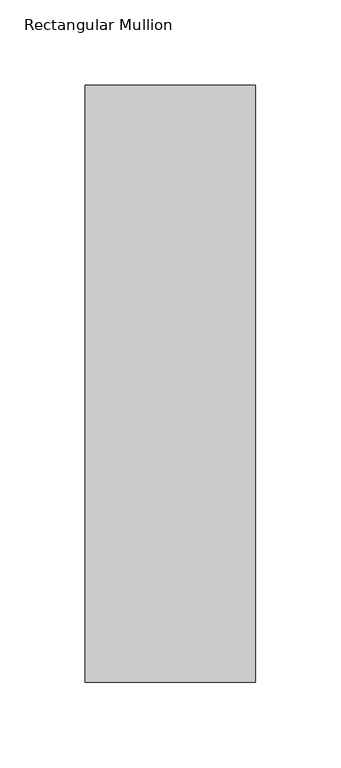
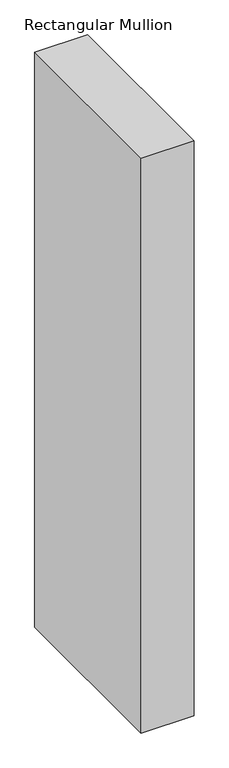
"""IFC4 building model written with IfcOpenShell, lengths in millimetres: member geometry, Rectangular Mullion : WWm-100x350-100mmOffset."""

import ifcopenshell
import ifcopenshell.guid

model = None  # the IFC model being written
_history = None  # IfcOwnerHistory: only IFC2X3 demands one
_inside = {}  # id of a spatial element -> (the spatial element, [elements in it])
_under = {}  # id of a project, library or spatial element -> (it, [spatial elements below it])
_declared = {}  # id of a project -> (the project, [libraries it declares])
_typed = {}  # id of a type object -> (the type object, [elements of that type])
_made_of = {}  # id of a material, layer set ... -> (it, [elements and type objects made of it])


def new_model(schema):
    """Start an empty IFC model of exactly this schema.

    Asked for "IFC4X3", IfcOpenShell would pick the latest addendum, in which some entities
    have other attributes; the version numbers below select the first issue.
    IFC2X3 requires an IfcOwnerHistory on every rooted entity: one is made here for all.
    """
    global model, _history
    if schema == "IFC4X3":
        model = ifcopenshell.file(schema_version=(4, 3, 0, 0))
    else:
        model = ifcopenshell.file(schema=schema)
    _inside.clear()
    _under.clear()
    _declared.clear()
    _typed.clear()
    _made_of.clear()
    _history = None
    if model.schema == "IFC2X3":
        org = make("IfcOrganization", Name="unknown")
        user = make(
            "IfcPersonAndOrganization",
            ThePerson=make("IfcPerson", FamilyName="unknown"),
            TheOrganization=org,
        )
        app = make(
            "IfcApplication",
            ApplicationDeveloper=org,
            Version="unknown",
            ApplicationFullName="unknown",
            ApplicationIdentifier="unknown",
        )
        _history = make(
            "IfcOwnerHistory",
            OwningUser=user,
            OwningApplication=app,
            ChangeAction="ADDED",
            CreationDate=0,
        )
    return model


def make(cls, **values):
    """One entity of the class cls with the attributes given. An attribute that is None is left unset."""
    return model.create_entity(
        cls, **{name: value for name, value in values.items() if value is not None}
    )


def rooted(cls, **values):
    """An entity with a GlobalId (a new one), such as an element, a storey or a relation."""
    return make(cls, GlobalId=ifcopenshell.guid.new(), OwnerHistory=_history, **values)


def si_unit(unit_type, name, prefix=None):
    """IfcSIUnit, for example si_unit("LENGTHUNIT", "METRE", prefix="MILLI")."""
    return make("IfcSIUnit", UnitType=unit_type, Prefix=prefix, Name=name)


def assignment(units):
    """IfcUnitAssignment: the units of a project."""
    return None if units is None else make("IfcUnitAssignment", Units=units)


def point(xyz):
    """IfcCartesianPoint."""
    return None if xyz is None else make("IfcCartesianPoint", Coordinates=xyz)


def direction(xyz):
    """IfcDirection."""
    return None if xyz is None else make("IfcDirection", DirectionRatios=xyz)


def frame(location, z_axis=None, x_axis=None):
    """IfcAxis2Placement3D, a coordinate frame: its origin and axes. An axis left out is left unset."""
    return make(
        "IfcAxis2Placement3D",
        Location=point(location),
        Axis=direction(z_axis),
        RefDirection=direction(x_axis),
    )


def origin():
    """The frame at (0, 0, 0) with its axes left unset."""
    return frame((0.0, 0.0, 0.0))


def place(relative_to, where):
    """IfcLocalPlacement: puts the frame where relative to a parent placement (None: the world)."""
    return make(
        "IfcLocalPlacement", PlacementRelTo=relative_to, RelativePlacement=where
    )


def context(
    kind, dimensions, precision=None, world=None, true_north=None, identifier=None
):
    """IfcGeometricRepresentationContext, for example the 3D "Model" context."""
    return make(
        "IfcGeometricRepresentationContext",
        ContextIdentifier=identifier,
        ContextType=kind,
        CoordinateSpaceDimension=dimensions,
        Precision=precision,
        WorldCoordinateSystem=world,
        TrueNorth=true_north,
    )


def project(units=None, contexts=None):
    """IfcProject with its units and contexts."""
    return rooted(
        "IfcProject",
        Name="project",
        RepresentationContexts=contexts,
        UnitsInContext=assignment(units),
    )


def spatial(cls, under=None, at=None, **own):
    """A site, building, storey or space (cls), placed at a placement, below another one or the project."""
    s = rooted(cls, ObjectPlacement=at, **own)
    if under is not None:
        _under.setdefault(under.id(), (under, []))[1].append(s)
    return s


def polyline(points):
    """IfcPolyline through the points."""
    return make("IfcPolyline", Points=[point(p) for p in points])


def outline(outer, holes=None, kind="AREA"):
    """IfcArbitraryClosedProfileDef: a profile drawn as a closed curve; with holes, ...WithVoids."""
    if holes is None:
        return make("IfcArbitraryClosedProfileDef", ProfileType=kind, OuterCurve=outer)
    return make(
        "IfcArbitraryProfileDefWithVoids",
        ProfileType=kind,
        OuterCurve=outer,
        InnerCurves=holes,
    )


def extrude(swept, where, along, depth):
    """IfcExtrudedAreaSolid: the profile swept, set in the frame where, extruded along a direction by depth."""
    return make(
        "IfcExtrudedAreaSolid",
        SweptArea=swept,
        Position=where,
        ExtrudedDirection=direction(along),
        Depth=depth,
    )


def shape(context_of_items, identifier, shape_type, items):
    """IfcShapeRepresentation: the items that make up one representation, for example the "Body"."""
    return make(
        "IfcShapeRepresentation",
        ContextOfItems=context_of_items,
        RepresentationIdentifier=identifier,
        RepresentationType=shape_type,
        Items=items,
    )


def source(mapping_origin, context_of_items, identifier, shape_type, items):
    """IfcRepresentationMap: a shape defined once, which mapped items show again and again."""
    return make(
        "IfcRepresentationMap",
        MappingOrigin=mapping_origin,
        MappedRepresentation=shape(context_of_items, identifier, shape_type, items),
    )


def transform(
    local_origin,
    x_axis=None,
    y_axis=None,
    z_axis=None,
    scale=None,
    scale2=None,
    scale3=None,
    uniform=True,
):
    """IfcCartesianTransformationOperator3D, or its non-uniform kind. x_axis, y_axis, z_axis: its Axis1, 2, 3."""
    if uniform:
        return make(
            "IfcCartesianTransformationOperator3D",
            Axis1=direction(x_axis),
            Axis2=direction(y_axis),
            LocalOrigin=point(local_origin),
            Scale=scale,
            Axis3=direction(z_axis),
        )
    return make(
        "IfcCartesianTransformationOperator3DnonUniform",
        Axis1=direction(x_axis),
        Axis2=direction(y_axis),
        LocalOrigin=point(local_origin),
        Scale=scale,
        Axis3=direction(z_axis),
        Scale2=scale2,
        Scale3=scale3,
    )


def mapped(mapping_source, mapping_target):
    """IfcMappedItem: shows the shape of a source again, moved by a transform."""
    return make(
        "IfcMappedItem", MappingSource=mapping_source, MappingTarget=mapping_target
    )


def made_of(thing, what):
    """Note that an element or type object is made of a material, layer set ...; save() writes the relation."""
    if what is not None:
        _made_of.setdefault(what.id(), (what, []))[1].append(thing)
    return thing


def element(
    cls,
    number,
    at=None,
    inside=None,
    cuts=None,
    type_object=None,
    material=None,
    context=None,
    identifier="Body",
    shape_type=None,
    held_by="IfcProductDefinitionShape",
    body=None,
    shapes=None,
    **own,
):
    """One element of the class cls, such as IfcWall. Its Tag is "e" and its number.

    at: its placement. inside: the storey or other place that contains it. cuts: it is an
    opening in that element (IfcRelVoidsElement). A single representation is given by context,
    identifier, shape_type and body (its items); several are given by shapes. held_by: the class
    of the entity that holds the representations. save() writes the other relations.
    """
    e = rooted(cls, Tag="e%d" % number, ObjectPlacement=at, **own)
    if body is not None:
        shapes = [shape(context, identifier, shape_type, body)]
    if shapes is not None:
        e.Representation = make(held_by, Representations=shapes)
    if inside is not None:
        _inside.setdefault(inside.id(), (inside, []))[1].append(e)
    if cuts is not None:
        rooted(
            "IfcRelVoidsElement", RelatingBuildingElement=cuts, RelatedOpeningElement=e
        )
    if type_object is not None:
        _typed.setdefault(type_object.id(), (type_object, []))[1].append(e)
    return made_of(e, material)


def aggregate(whole, parts):
    """IfcRelAggregates: a whole, such as a stair, and the parts it consists of."""
    return rooted("IfcRelAggregates", RelatingObject=whole, RelatedObjects=parts)


def save(model, path):
    """Write the relations noted so far, then the file.

    IfcRelAggregates (storeys below a building ...), IfcRelContainedInSpatialStructure (elements
    in a storey), IfcRelDefinesByType, IfcRelAssociatesMaterial and IfcRelDeclares: one each for
    every whole, place, type object, material and project.
    """
    for whole, parts in _under.values():
        aggregate(whole, parts)
    for where, things in _inside.values():
        rooted(
            "IfcRelContainedInSpatialStructure",
            RelatedElements=things,
            RelatingStructure=where,
        )
    for kind, things in _typed.values():
        rooted("IfcRelDefinesByType", RelatedObjects=things, RelatingType=kind)
    for what, things in _made_of.values():
        rooted("IfcRelAssociatesMaterial", RelatedObjects=things, RelatingMaterial=what)
    for by, libraries in _declared.values():
        rooted("IfcRelDeclares", RelatingContext=by, RelatedDefinitions=libraries)
    model.write(path)


def rectangular_mullion_77d02227(model_context):
    return source(origin(), model_context, "Body", "SweptSolid", [
        extrude(outline(polyline([(0.0, 175.0), (0.0, -175.0), (-100.0, -175.0), (-100.0, 175.0), (0.0, 175.0)])), frame((0.0, 0.0, -1152.7090118), z_axis=(0.0, 0.0, 1.0), x_axis=(1.0, 0.0, 0.0)), (0.0, 0.0, 1.0), 1152.7090118),
    ])


if __name__ == "__main__":
    model = new_model("IFC4")
    model_context = context("Model", 3, world=origin())
    ifc_project = project(units=[si_unit("LENGTHUNIT", "METRE", prefix="MILLI")], contexts=[model_context])
    site = spatial("IfcSite", under=ifc_project)
    building = spatial("IfcBuilding", under=site)
    placement = place(None, origin())
    rectangular_mullion_shape = rectangular_mullion_77d02227(model_context)
    element("IfcMember", 1, ObjectType="Rectangular Mullion : WWm-100x350-100mmOffset", at=placement, inside=building, context=model_context, shape_type="MappedRepresentation", body=[
        mapped(rectangular_mullion_shape, transform((0.0, 0.0, 0.0), x_axis=(1.0, 0.0, 0.0), y_axis=(0.0, 1.0, 0.0), z_axis=(0.0, 0.0, 1.0))),
    ])
    save(model, "model.ifc")

# Revit data of these elements
# Type "Rectangular Mullion : WWm-100x350-100mmOffset"
#   built-in parameter 1007304 = 1.14829 (stored number, unit not read)
#   built-in parameter 1007301 = 0.164042 (stored number, unit not read)
#   built-in parameter 1007300 = 0.164042 (stored number, unit not read)
# Element 1 (IfcMember, "Rectangular Mullion : WWm-100x350-100mmOffset")
#   Materials on its faces: "WW-EC-RGB-Mullion"
# Materials
#   "WW-EC-RGB-Mullion": class "Generic", colour RGB 255 255 255, transparency 0, Comments = "If region requests black mullions, switch asset color to RGB 25-25-25", Description = "Generic Color", Cost = 0
